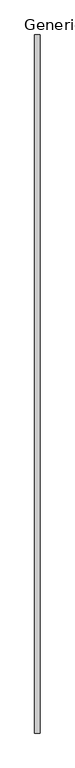
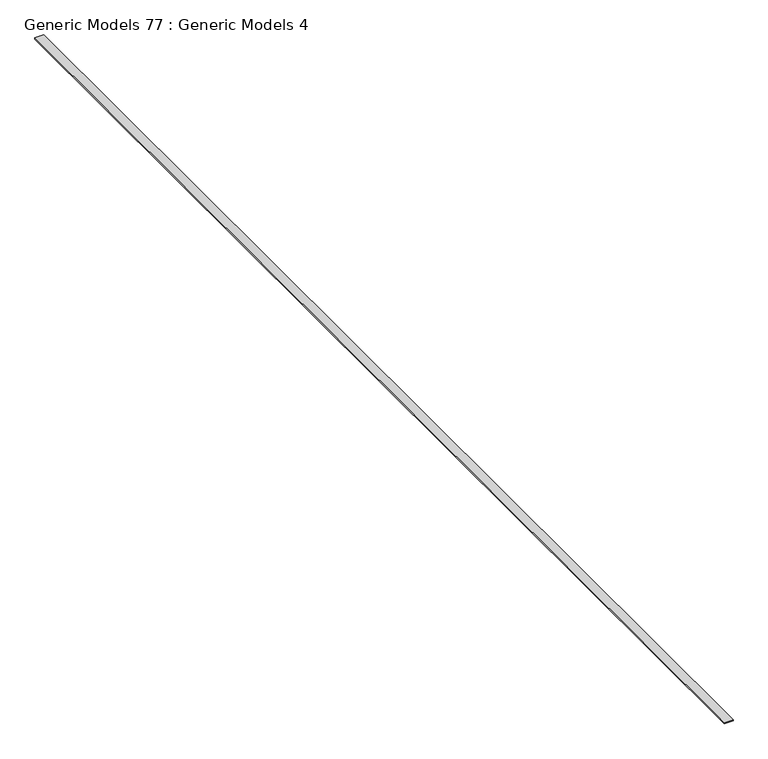
"""IFC4 building model written with IfcOpenShell, lengths in millimetres: proxy geometry, Generic Models 77 : Generic Models 4."""

from ifc_helpers import new_model, si_unit, frame, origin, place, context, project, spatial, polyline, outline, extrude, source, transform, mapped, element, save


def generic_models_77_generic_models_4_277462be(model_context):
    return source(origin(), model_context, "Body", "SweptSolid", [
        extrude(outline(polyline([(-8185.3236295, -6864.9230338), (-8325.0236295, -6864.9230338), (-8325.0236295, 11778.6769662), (-8185.3236295, 11778.6769662), (-8185.3236295, -6864.9230338)])), frame((0.0, 0.0, 126806.071), z_axis=(0.0, 0.0, 1.0), x_axis=(1.0, 0.0, 0.0)), (0.0, 0.0, 1.0), 22.225),
    ])


if __name__ == "__main__":
    model = new_model("IFC4")
    model_context = context("Model", 3, world=origin())
    ifc_project = project(units=[si_unit("LENGTHUNIT", "METRE", prefix="MILLI")], contexts=[model_context])
    site = spatial("IfcSite", under=ifc_project)
    building = spatial("IfcBuilding", under=site)
    placement = place(None, origin())
    generic_models_77_generic_models_4_shape = generic_models_77_generic_models_4_277462be(model_context)
    element("IfcBuildingElementProxy", 1, Name="Generic Models 77 : Generic Models 4", ObjectType="Generic Models 77 : Generic Models 4", at=placement, inside=building, context=model_context, shape_type="MappedRepresentation", body=[
        mapped(generic_models_77_generic_models_4_shape, transform((0.0, 0.0, 0.0), x_axis=(1.0, 0.0, 0.0), y_axis=(0.0, 1.0, 0.0), z_axis=(0.0, 0.0, 1.0))),
    ])
    save(model, "model.ifc")

# Revit data of these elements
# Element 1 (IfcBuildingElementProxy, "Generic Models 77 : Generic Models 4")
#   Materials on its faces: "_2X BLOCKING AS REQUIRED"
# Materials
#   "_2X BLOCKING AS REQUIRED": class "Generic", colour RGB 177 130 114, transparency 0, Cost = 0
